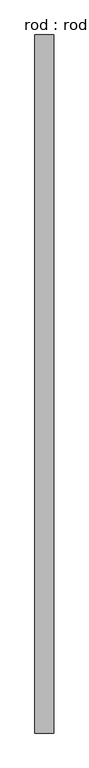
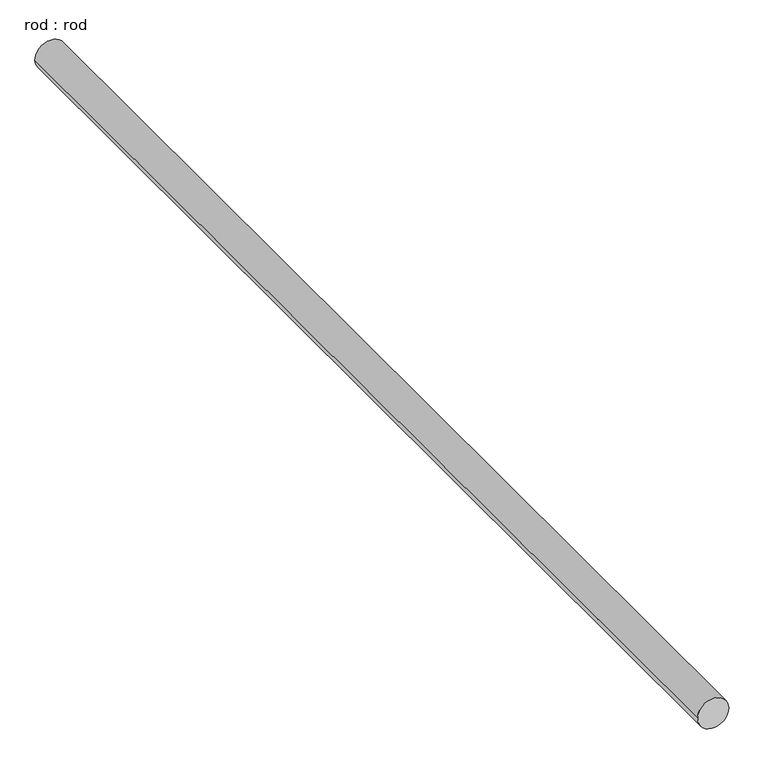
"""IFC4 building model written with IfcOpenShell, lengths in millimetres: proxy geometry, rod : rod."""

from ifc_helpers import new_model, si_unit, point, frame, frame_2d, origin, place, context, project, spatial, circle_curve, trimmed, segment, composite_curve, outline, extrude, source, transform, mapped, element, save


def rod_rod_c016f796(model_context):
    return source(origin(), model_context, "Body", "SweptSolid", [
        extrude(outline(composite_curve([segment(trimmed(circle_curve(frame_2d((0.0108462, 0.0)), 200.0), [point((0.0108462, 200.0))], [point((0.0108462, -200.0))], False, "CARTESIAN"), True, "CONTINUOUS"), segment(trimmed(circle_curve(frame_2d((0.0108462, 0.0)), 200.0), [point((0.0108462, -200.0))], [point((0.0108462, 200.0))], False, "CARTESIAN"), True, "CONTINUOUS")], self_intersect=False)), frame((0.0, -3259.9499561, 0.0), z_axis=(0.0, 1.0, 0.0), x_axis=(0.0, 0.0, 1.0)), (0.0, 0.0, 1.0), 14705.3571429),
    ])


if __name__ == "__main__":
    model = new_model("IFC4")
    model_context = context("Model", 3, world=origin())
    ifc_project = project(units=[si_unit("LENGTHUNIT", "METRE", prefix="MILLI")], contexts=[model_context])
    site = spatial("IfcSite", under=ifc_project)
    building = spatial("IfcBuilding", under=site)
    placement = place(None, origin())
    rod_rod_shape = rod_rod_c016f796(model_context)
    element("IfcBuildingElementProxy", 1, Name="rod : rod", ObjectType="rod : rod", at=placement, inside=building, context=model_context, shape_type="MappedRepresentation", body=[
        mapped(rod_rod_shape, transform((0.0, 0.0, 0.0), x_axis=(1.0, 0.0, 0.0), y_axis=(0.0, 1.0, 0.0), z_axis=(0.0, 0.0, 1.0))),
    ])
    save(model, "model.ifc")

# Revit data of these elements
# Type "rod : rod"
#   Default Elevation = 0
